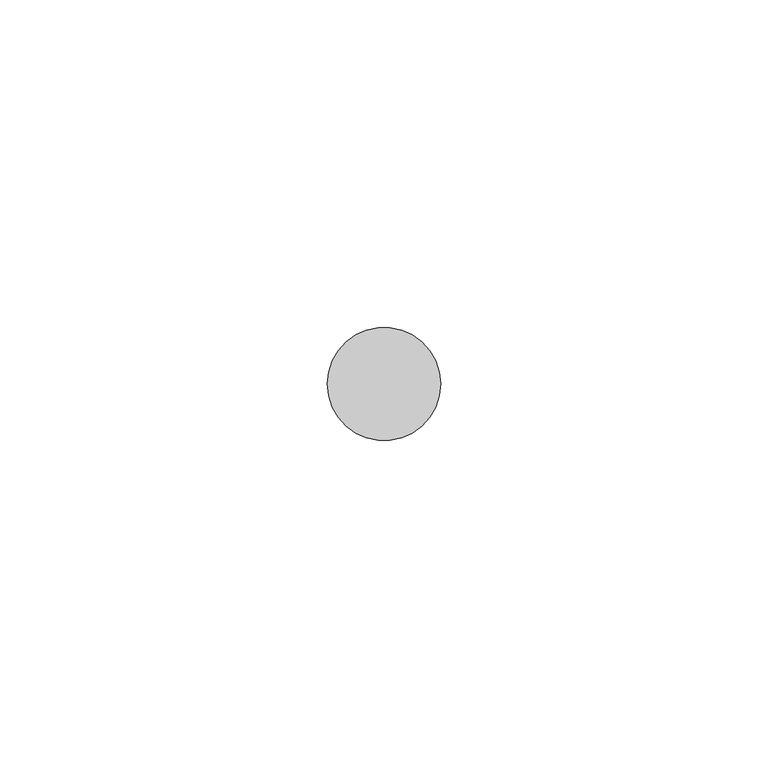
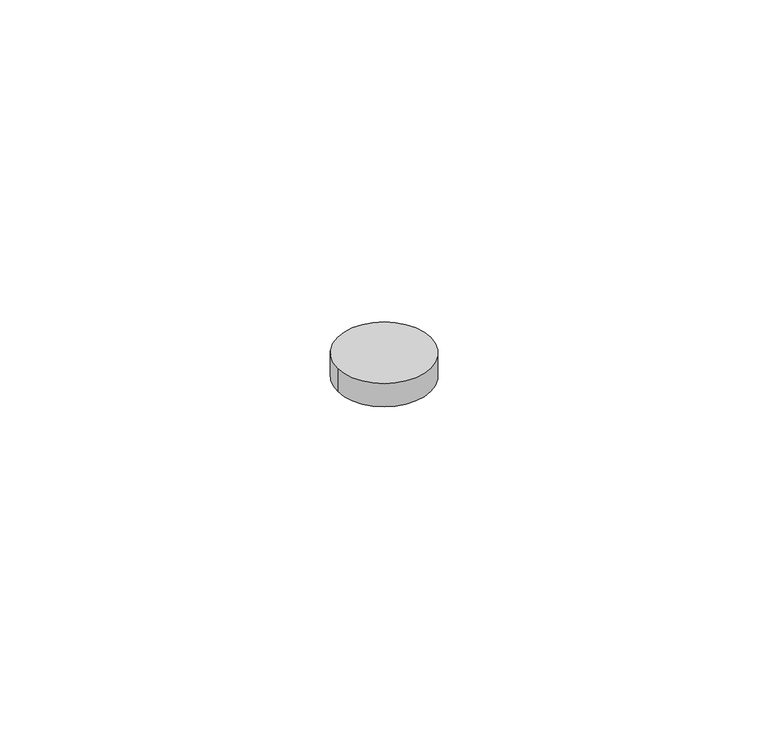
"""IFC4 building model written with IfcOpenShell, lengths in millimetres: proxy geometry, Hinge Pin Keeper11 : Hinge Pin Keeper."""

from ifc_helpers import new_model, si_unit, point, frame, frame_2d, origin, place, context, project, spatial, circle_curve, trimmed, segment, composite_curve, outline, extrude, source, transform, mapped, element, save


def generic_models_2922e777(model_context):
    return source(origin(), model_context, "Body", "SweptSolid", [
        extrude(outline(composite_curve([segment(trimmed(circle_curve(frame_2d((587319.1320739, -536310.3652841)), 8.6534625), [point((587310.4786114, -536310.3652841))], [point((587327.7855364, -536310.3652841))], False, "CARTESIAN"), True, "CONTINUOUS"), segment(trimmed(circle_curve(frame_2d((587319.1320739, -536310.3652841)), 8.6534625), [point((587327.7855364, -536310.3652841))], [point((587310.4786114, -536310.3652841))], False, "CARTESIAN"), True, "CONTINUOUS")], self_intersect=False)), frame((0.0, 0.0, 1271.7859375), z_axis=(0.0, 0.0, 1.0), x_axis=(1.0, 0.0, 0.0)), (0.0, 0.0, 1.0), 4.5640625),
    ])


if __name__ == "__main__":
    model = new_model("IFC4")
    model_context = context("Model", 3, world=origin())
    ifc_project = project(units=[si_unit("LENGTHUNIT", "METRE", prefix="MILLI")], contexts=[model_context])
    site = spatial("IfcSite", under=ifc_project)
    building = spatial("IfcBuilding", under=site)
    placement = place(None, origin())
    generic_models_shape = generic_models_2922e777(model_context)
    element("IfcBuildingElementProxy", 1, Name="Hinge Pin Keeper11 : Hinge Pin Keeper", ObjectType="Hinge Pin Keeper11 : Hinge Pin Keeper", at=placement, inside=building, context=model_context, shape_type="MappedRepresentation", body=[
        mapped(generic_models_shape, transform((0.0, 0.0, 0.0), x_axis=(1.0, 0.0, 0.0), y_axis=(0.0, 1.0, 0.0), z_axis=(0.0, 0.0, 1.0))),
    ])
    save(model, "model.ifc")

# Revit data of these elements
# Element 1 (IfcBuildingElementProxy, "Hinge Pin Keeper11 : Hinge Pin Keeper")
#   Materials on its faces: "6\"X6\" WELD-ON STL BUTT HINGE"
# Materials
#   "6\"X6\" WELD-ON STL BUTT HINGE": class "Metal", colour RGB 189 187 185, transparency 0, Description = "Carbon steel", Cost = 0
